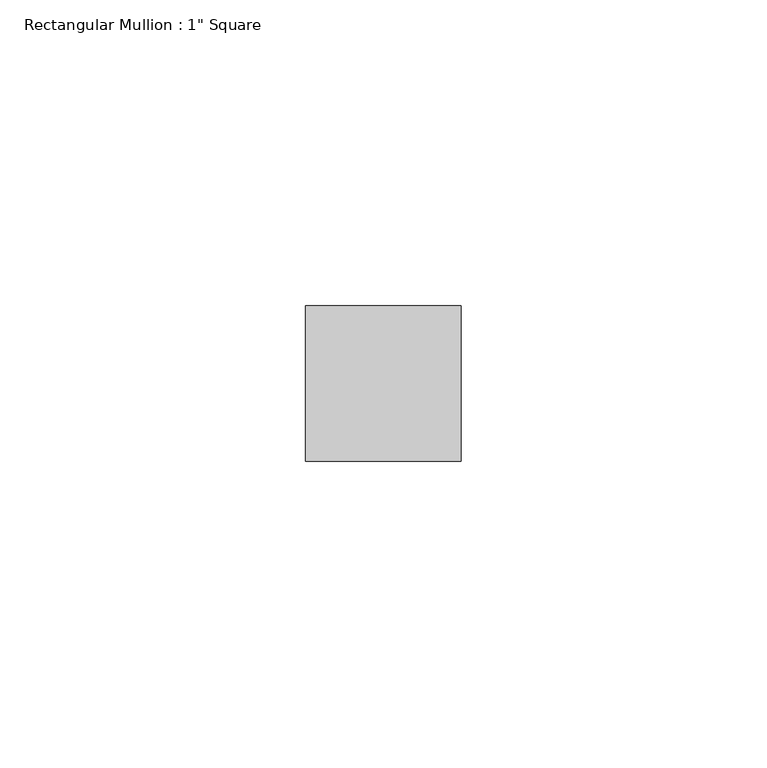
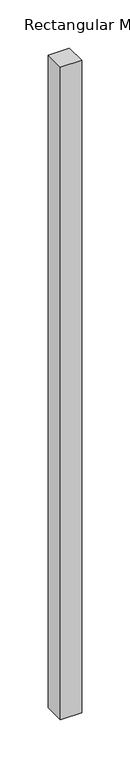
"""IFC4 building model written with IfcOpenShell, lengths in millimetres: member geometry."""

from ifc_helpers import new_model, si_unit, frame, origin, place, context, project, spatial, polyline, outline, extrude, source, transform, mapped, element, save


def member_f95b3a9c(model_context):
    return source(origin(), model_context, "Body", "SweptSolid", [
        extrude(outline(polyline([(12.7, 12.7), (12.7, -12.7), (-12.7, -12.7), (-12.7, 12.7), (12.7, 12.7)])), frame((0.0, 0.0, -825.5), z_axis=(0.0, 0.0, 1.0), x_axis=(1.0, 0.0, 0.0)), (0.0, 0.0, 1.0), 825.5),
    ])


if __name__ == "__main__":
    model = new_model("IFC4")
    model_context = context("Model", 3, world=origin())
    ifc_project = project(units=[si_unit("LENGTHUNIT", "METRE", prefix="MILLI")], contexts=[model_context])
    site = spatial("IfcSite", under=ifc_project)
    building = spatial("IfcBuilding", under=site)
    placement = place(None, origin())
    member_shape = member_f95b3a9c(model_context)
    element("IfcMember", 1, ObjectType="Rectangular Mullion : 1\" Square", at=placement, inside=building, context=model_context, shape_type="MappedRepresentation", body=[
        mapped(member_shape, transform((0.0, 0.0, 0.0), x_axis=(1.0, 0.0, 0.0), y_axis=(0.0, 1.0, 0.0), z_axis=(0.0, 0.0, 1.0))),
    ])
    save(model, "model.ifc")

# Revit data of these elements
# Type "Rectangular Mullion : 1\" Square"
#   built-in parameter 1007304 = 0.0833333 (stored number, unit not read)
#   built-in parameter 1007301 = 0.0416667 (stored number, unit not read)
#   built-in parameter 1007300 = 0.0416667 (stored number, unit not read)
# Element 1 (IfcMember, "Rectangular Mullion : 1\" Square")
#   Materials on its faces: "Metal - Aluminum"
# Materials
#   "Metal - Aluminum": class "Metal", colour RGB 247 247 247, transparency 0
